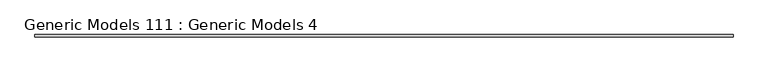
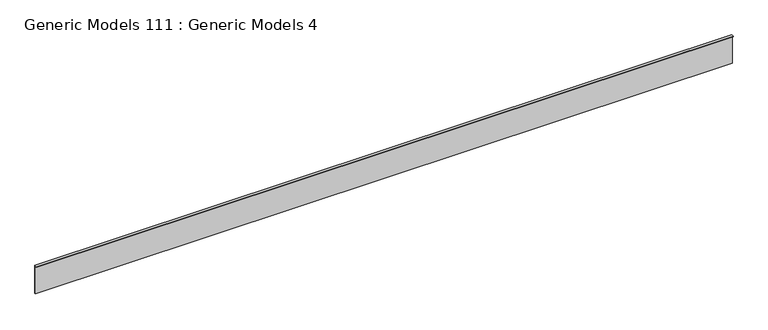
"""IFC4 building model written with IfcOpenShell, lengths in millimetres: proxy geometry, Generic Models 111 : Generic Models 4."""

from ifc_helpers import new_model, si_unit, frame, origin, place, context, project, spatial, polyline, outline, extrude, source, transform, mapped, element, save


def generic_models_111_generic_models_4_23b71d15(model_context):
    return source(origin(), model_context, "Body", "SweptSolid", [
        extrude(outline(polyline([(7036.0769221, 123424.696), (7036.0769221, 124205.0900166), (6990.9493503, 124205.0900166), (6990.9493503, 124222.5525166), (7053.8569221, 124222.5525166), (7053.8569221, 123424.696), (7036.0769221, 123424.696)])), frame((-10259.9171316, 0.0, 0.0), z_axis=(1.0, 0.0, 0.0), x_axis=(0.0, 1.0, 0.0)), (0.0, 0.0, 1.0), 18643.6),
    ])


if __name__ == "__main__":
    model = new_model("IFC4")
    model_context = context("Model", 3, world=origin())
    ifc_project = project(units=[si_unit("LENGTHUNIT", "METRE", prefix="MILLI")], contexts=[model_context])
    site = spatial("IfcSite", under=ifc_project)
    building = spatial("IfcBuilding", under=site)
    placement = place(None, origin())
    generic_models_111_generic_models_4_shape = generic_models_111_generic_models_4_23b71d15(model_context)
    element("IfcBuildingElementProxy", 1, Name="Generic Models 111 : Generic Models 4", ObjectType="Generic Models 111 : Generic Models 4", at=placement, inside=building, context=model_context, shape_type="MappedRepresentation", body=[
        mapped(generic_models_111_generic_models_4_shape, transform((0.0, 0.0, 0.0), x_axis=(1.0, 0.0, 0.0), y_axis=(0.0, 1.0, 0.0), z_axis=(0.0, 0.0, 1.0))),
    ])
    save(model, "model.ifc")

# Revit data of these elements
# Element 1 (IfcBuildingElementProxy, "Generic Models 111 : Generic Models 4")
#   Materials on its faces: "_5/8\" GYPSUM BOARD, PAINTED"
# Materials
#   "_5/8\" GYPSUM BOARD, PAINTED": class "Generic", colour RGB 233 233 233, transparency 0, Cost = 0
